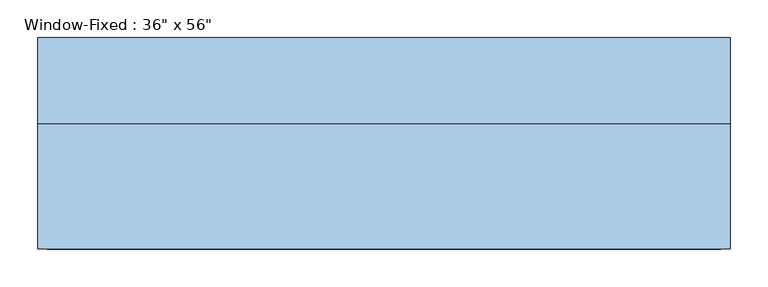
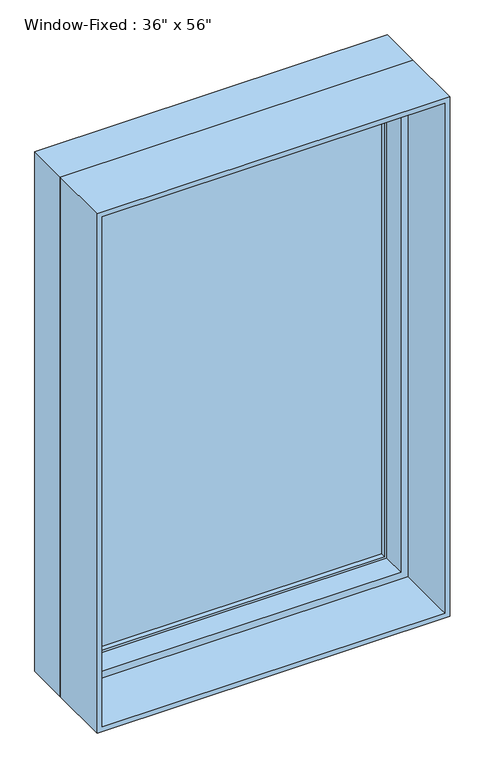
"""IFC4 building model written with IfcOpenShell, lengths in millimetres: window geometry."""

import ifcopenshell
import ifcopenshell.guid

model = None  # the IFC model being written
_history = None  # IfcOwnerHistory: only IFC2X3 demands one
_inside = {}  # id of a spatial element -> (the spatial element, [elements in it])
_under = {}  # id of a project, library or spatial element -> (it, [spatial elements below it])
_declared = {}  # id of a project -> (the project, [libraries it declares])
_typed = {}  # id of a type object -> (the type object, [elements of that type])
_made_of = {}  # id of a material, layer set ... -> (it, [elements and type objects made of it])


def new_model(schema):
    """Start an empty IFC model of exactly this schema.

    Asked for "IFC4X3", IfcOpenShell would pick the latest addendum, in which some entities
    have other attributes; the version numbers below select the first issue.
    IFC2X3 requires an IfcOwnerHistory on every rooted entity: one is made here for all.
    """
    global model, _history
    if schema == "IFC4X3":
        model = ifcopenshell.file(schema_version=(4, 3, 0, 0))
    else:
        model = ifcopenshell.file(schema=schema)
    _inside.clear()
    _under.clear()
    _declared.clear()
    _typed.clear()
    _made_of.clear()
    _history = None
    if model.schema == "IFC2X3":
        org = make("IfcOrganization", Name="unknown")
        user = make(
            "IfcPersonAndOrganization",
            ThePerson=make("IfcPerson", FamilyName="unknown"),
            TheOrganization=org,
        )
        app = make(
            "IfcApplication",
            ApplicationDeveloper=org,
            Version="unknown",
            ApplicationFullName="unknown",
            ApplicationIdentifier="unknown",
        )
        _history = make(
            "IfcOwnerHistory",
            OwningUser=user,
            OwningApplication=app,
            ChangeAction="ADDED",
            CreationDate=0,
        )
    return model


def make(cls, **values):
    """One entity of the class cls with the attributes given. An attribute that is None is left unset."""
    return model.create_entity(
        cls, **{name: value for name, value in values.items() if value is not None}
    )


def rooted(cls, **values):
    """An entity with a GlobalId (a new one), such as an element, a storey or a relation."""
    return make(cls, GlobalId=ifcopenshell.guid.new(), OwnerHistory=_history, **values)


def si_unit(unit_type, name, prefix=None):
    """IfcSIUnit, for example si_unit("LENGTHUNIT", "METRE", prefix="MILLI")."""
    return make("IfcSIUnit", UnitType=unit_type, Prefix=prefix, Name=name)


def assignment(units):
    """IfcUnitAssignment: the units of a project."""
    return None if units is None else make("IfcUnitAssignment", Units=units)


def point(xyz):
    """IfcCartesianPoint."""
    return None if xyz is None else make("IfcCartesianPoint", Coordinates=xyz)


def direction(xyz):
    """IfcDirection."""
    return None if xyz is None else make("IfcDirection", DirectionRatios=xyz)


def frame(location, z_axis=None, x_axis=None):
    """IfcAxis2Placement3D, a coordinate frame: its origin and axes. An axis left out is left unset."""
    return make(
        "IfcAxis2Placement3D",
        Location=point(location),
        Axis=direction(z_axis),
        RefDirection=direction(x_axis),
    )


def origin():
    """The frame at (0, 0, 0) with its axes left unset."""
    return frame((0.0, 0.0, 0.0))


def place(relative_to, where):
    """IfcLocalPlacement: puts the frame where relative to a parent placement (None: the world)."""
    return make(
        "IfcLocalPlacement", PlacementRelTo=relative_to, RelativePlacement=where
    )


def context(
    kind, dimensions, precision=None, world=None, true_north=None, identifier=None
):
    """IfcGeometricRepresentationContext, for example the 3D "Model" context."""
    return make(
        "IfcGeometricRepresentationContext",
        ContextIdentifier=identifier,
        ContextType=kind,
        CoordinateSpaceDimension=dimensions,
        Precision=precision,
        WorldCoordinateSystem=world,
        TrueNorth=true_north,
    )


def project(units=None, contexts=None):
    """IfcProject with its units and contexts."""
    return rooted(
        "IfcProject",
        Name="project",
        RepresentationContexts=contexts,
        UnitsInContext=assignment(units),
    )


def spatial(cls, under=None, at=None, **own):
    """A site, building, storey or space (cls), placed at a placement, below another one or the project."""
    s = rooted(cls, ObjectPlacement=at, **own)
    if under is not None:
        _under.setdefault(under.id(), (under, []))[1].append(s)
    return s


def polyline(points):
    """IfcPolyline through the points."""
    return make("IfcPolyline", Points=[point(p) for p in points])


def outline(outer, holes=None, kind="AREA"):
    """IfcArbitraryClosedProfileDef: a profile drawn as a closed curve; with holes, ...WithVoids."""
    if holes is None:
        return make("IfcArbitraryClosedProfileDef", ProfileType=kind, OuterCurve=outer)
    return make(
        "IfcArbitraryProfileDefWithVoids",
        ProfileType=kind,
        OuterCurve=outer,
        InnerCurves=holes,
    )


def extrude(swept, where, along, depth):
    """IfcExtrudedAreaSolid: the profile swept, set in the frame where, extruded along a direction by depth."""
    return make(
        "IfcExtrudedAreaSolid",
        SweptArea=swept,
        Position=where,
        ExtrudedDirection=direction(along),
        Depth=depth,
    )


def faces_of(points, faces, orient=None, outer=None):
    """IfcFace entities. A face is a list of loops; a loop is a list of indices into points, from 0.

    orient and outer hold one flag for each loop. By default every Orientation is true, the
    first loop of a face is its IfcFaceOuterBound and the others are IfcFaceBound.
    """
    made = []
    for i, loops in enumerate(faces):
        bounds = []
        for j, loop in enumerate(loops):
            is_outer = j == 0 if outer is None else outer[i][j]
            bounds.append(
                make(
                    "IfcFaceOuterBound" if is_outer else "IfcFaceBound",
                    Bound=make("IfcPolyLoop", Polygon=[points[k] for k in loop]),
                    Orientation=True if orient is None else orient[i][j],
                )
            )
        made.append(make("IfcFace", Bounds=bounds))
    return made


def faceted_brep(points, faces, orient=None, outer=None, voids=None):
    """IfcFacetedBrep: a solid bounded by flat faces; with voids (closed shells), ...WithVoids."""
    shared = [point(p) for p in points]
    hull = make("IfcClosedShell", CfsFaces=faces_of(shared, faces, orient, outer))
    if voids is None:
        return make("IfcFacetedBrep", Outer=hull)
    return make(
        "IfcFacetedBrepWithVoids",
        Outer=hull,
        Voids=[
            make(cls, CfsFaces=faces_of(shared, fs, o, b)) for cls, fs, o, b in voids
        ],
    )


def shape(context_of_items, identifier, shape_type, items):
    """IfcShapeRepresentation: the items that make up one representation, for example the "Body"."""
    return make(
        "IfcShapeRepresentation",
        ContextOfItems=context_of_items,
        RepresentationIdentifier=identifier,
        RepresentationType=shape_type,
        Items=items,
    )


def source(mapping_origin, context_of_items, identifier, shape_type, items):
    """IfcRepresentationMap: a shape defined once, which mapped items show again and again."""
    return make(
        "IfcRepresentationMap",
        MappingOrigin=mapping_origin,
        MappedRepresentation=shape(context_of_items, identifier, shape_type, items),
    )


def transform(
    local_origin,
    x_axis=None,
    y_axis=None,
    z_axis=None,
    scale=None,
    scale2=None,
    scale3=None,
    uniform=True,
):
    """IfcCartesianTransformationOperator3D, or its non-uniform kind. x_axis, y_axis, z_axis: its Axis1, 2, 3."""
    if uniform:
        return make(
            "IfcCartesianTransformationOperator3D",
            Axis1=direction(x_axis),
            Axis2=direction(y_axis),
            LocalOrigin=point(local_origin),
            Scale=scale,
            Axis3=direction(z_axis),
        )
    return make(
        "IfcCartesianTransformationOperator3DnonUniform",
        Axis1=direction(x_axis),
        Axis2=direction(y_axis),
        LocalOrigin=point(local_origin),
        Scale=scale,
        Axis3=direction(z_axis),
        Scale2=scale2,
        Scale3=scale3,
    )


def mapped(mapping_source, mapping_target):
    """IfcMappedItem: shows the shape of a source again, moved by a transform."""
    return make(
        "IfcMappedItem", MappingSource=mapping_source, MappingTarget=mapping_target
    )


def made_of(thing, what):
    """Note that an element or type object is made of a material, layer set ...; save() writes the relation."""
    if what is not None:
        _made_of.setdefault(what.id(), (what, []))[1].append(thing)
    return thing


def element(
    cls,
    number,
    at=None,
    inside=None,
    cuts=None,
    type_object=None,
    material=None,
    context=None,
    identifier="Body",
    shape_type=None,
    held_by="IfcProductDefinitionShape",
    body=None,
    shapes=None,
    **own,
):
    """One element of the class cls, such as IfcWall. Its Tag is "e" and its number.

    at: its placement. inside: the storey or other place that contains it. cuts: it is an
    opening in that element (IfcRelVoidsElement). A single representation is given by context,
    identifier, shape_type and body (its items); several are given by shapes. held_by: the class
    of the entity that holds the representations. save() writes the other relations.
    """
    e = rooted(cls, Tag="e%d" % number, ObjectPlacement=at, **own)
    if body is not None:
        shapes = [shape(context, identifier, shape_type, body)]
    if shapes is not None:
        e.Representation = make(held_by, Representations=shapes)
    if inside is not None:
        _inside.setdefault(inside.id(), (inside, []))[1].append(e)
    if cuts is not None:
        rooted(
            "IfcRelVoidsElement", RelatingBuildingElement=cuts, RelatedOpeningElement=e
        )
    if type_object is not None:
        _typed.setdefault(type_object.id(), (type_object, []))[1].append(e)
    return made_of(e, material)


def aggregate(whole, parts):
    """IfcRelAggregates: a whole, such as a stair, and the parts it consists of."""
    return rooted("IfcRelAggregates", RelatingObject=whole, RelatedObjects=parts)


def save(model, path):
    """Write the relations noted so far, then the file.

    IfcRelAggregates (storeys below a building ...), IfcRelContainedInSpatialStructure (elements
    in a storey), IfcRelDefinesByType, IfcRelAssociatesMaterial and IfcRelDeclares: one each for
    every whole, place, type object, material and project.
    """
    for whole, parts in _under.values():
        aggregate(whole, parts)
    for where, things in _inside.values():
        rooted(
            "IfcRelContainedInSpatialStructure",
            RelatedElements=things,
            RelatingStructure=where,
        )
    for kind, things in _typed.values():
        rooted("IfcRelDefinesByType", RelatedObjects=things, RelatingType=kind)
    for what, things in _made_of.values():
        rooted("IfcRelAssociatesMaterial", RelatedObjects=things, RelatingMaterial=what)
    for by, libraries in _declared.values():
        rooted("IfcRelDeclares", RelatingContext=by, RelatedDefinitions=libraries)
    model.write(path)


def window_fe4c84aa(model_context):
    return source(origin(), model_context, "Body", "SolidModel", [
        extrude(outline(polyline([(419.1, 104.775), (419.1, 98.425), (-419.1, 98.425), (-419.1, 104.775), (419.1, 104.775)])), frame((0.0, 0.0, 952.5), z_axis=(0.0, 0.0, 1.0), x_axis=(1.0, 0.0, 0.0)), (0.0, 0.0, 1.0), 1346.2),
        extrude(outline(polyline([(-419.1, 85.725), (-419.1, 92.075), (419.1, 92.075), (419.1, 85.725), (-419.1, 85.725)])), frame((0.0, 0.0, 952.5), z_axis=(0.0, 0.0, 1.0), x_axis=(1.0, 0.0, 0.0)), (0.0, 0.0, 1.0), 1346.2),
        extrude(outline(polyline([(927.1, 444.5), (2324.1, 444.5), (2324.1, -444.5), (927.1, -444.5), (927.1, 444.5)]), holes=[polyline([(952.5, -419.1), (2298.7, -419.1), (2298.7, 419.1), (952.5, 419.1), (952.5, -419.1)])]), frame((0.0, 73.025, 0.0), z_axis=(0.0, 1.0, 0.0), x_axis=(0.0, 0.0, 1.0)), (0.0, 0.0, 1.0), 44.45),
        extrude(outline(polyline([(2336.8, -457.2), (914.4, -457.2), (914.4, 457.2), (2336.8, 457.2), (2336.8, -457.2)]), holes=[polyline([(2324.1, 444.5), (927.1, 444.5), (927.1, -444.5), (2324.1, -444.5), (2324.1, 444.5)])]), frame((0.0, -155.575, 0.0), z_axis=(0.0, 1.0, 0.0), x_axis=(0.0, 0.0, 1.0)), (0.0, 0.0, 1.0), 165.1),
        faceted_brep([(457.2, 9.525, 2336.8), (457.2, 123.825, 2336.8), (-457.2, 123.825, 2336.8), (-457.2, 9.525, 2336.8), (-457.2, 123.825, 914.4), (-457.2, 9.525, 914.4), (457.2, 123.825, 914.4), (457.2, 9.525, 914.4), (425.45, 9.525, 2305.05), (425.45, 9.525, 946.15), (-425.45, 9.525, 946.15), (-425.45, 9.525, 2305.05), (-444.5, 123.825, 2324.1), (-444.5, 123.825, 927.1), (444.5, 123.825, 927.1), (444.5, 123.825, 2324.1), (425.45, 73.025, 2305.05), (-425.45, 73.025, 2305.05), (444.5, 73.025, 2324.1), (-444.5, 73.025, 2324.1), (-425.45, 73.025, 946.15), (-444.5, 73.025, 927.1), (425.45, 73.025, 946.15), (444.5, 73.025, 927.1)], [[[0, 1, 2, 3]], [[3, 2, 4, 5]], [[5, 4, 6, 7]], [[3, 5, 7, 0], [8, 9, 10, 11]], [[7, 6, 1, 0]], [[1, 6, 4, 2], [12, 13, 14, 15]], [[16, 8, 11, 17]], [[15, 18, 19, 12]], [[17, 11, 10, 20]], [[12, 19, 21, 13]], [[20, 10, 9, 22]], [[13, 21, 23, 14]], [[22, 9, 8, 16]], [[18, 23, 21, 19], [17, 20, 22, 16]], [[14, 23, 18, 15]]]),
    ])


if __name__ == "__main__":
    model = new_model("IFC4")
    model_context = context("Model", 3, world=origin())
    ifc_project = project(units=[si_unit("LENGTHUNIT", "METRE", prefix="MILLI")], contexts=[model_context])
    site = spatial("IfcSite", under=ifc_project)
    building = spatial("IfcBuilding", under=site)
    placement = place(None, origin())
    window_shape = window_fe4c84aa(model_context)
    element("IfcWindow", 1, ObjectType="Window-Fixed : 36\" x 56\"", at=placement, inside=building, context=model_context, shape_type="MappedRepresentation", body=[
        mapped(window_shape, transform((0.0, 0.0, 0.0), x_axis=(1.0, 0.0, 0.0), y_axis=(0.0, 1.0, 0.0), z_axis=(0.0, 0.0, 1.0))),
    ])
    save(model, "model.ifc")

# Revit data of these elements
# Type "Window-Fixed : 36\" x 56\""
#   Type Mark = "22"
#   Fire Rating = "0.5h"
#   Assembly Code = "B2020100"
#   Analytic Construction = "Double glazing - domestic"
#   Window Inset [instance default] = 0' - 0"
#   Wall Thickness [instance default] = 0' - 6"
#   Visual Light Transmittance = 0.81
#   Thermal Resistance (R) = 1.8146 (h·ft²·°F)/BTU
#   Solar Heat Gain Coefficient = 0.76
#   Rough Width = 3' - 0 1/2"
#   Rough Height = 4' - 8 1/2"
#   Interior Wall Closure [instance default] = 0' - 2 1/4"
#   Height = 4' - 8"
#   Heat Transfer Coefficient (U) = 0.5511 BTU/(h·ft²·°F)
#   Frame Extension [instance default] = 0' - 0 1/4"
#   Exterior Wall Closure [instance default] = 0' - 1 1/4"
#   Extension Jamb [instance default] = 0' - 2 1/4"
#   Default Sill Height = 3' - 0"
#   Width = 3' - 0"
#   Muntin Visibility = yes
#   Interior Trim Visibility [instance default] = yes
#   Exterior Trim Visibility [instance default] = yes
#   Extension Jamb Visibility [instance default] = yes
#   Muntin Pattern = Muntin Pattern_2x2 : Muntin Pattern_2x2
#   Interior Trim Material = Wood - Stained
#   Interior Trim = Trim-Window-Interior-Flat : Picture Frame
#   Interior Frame Material = Wood - Stained
#   Glass Panel Material = Glass
#   Exterior Trim Material = Clad - White
#   Exterior Trim = Trim-Window-Exterior-Flat : with Sill
#   Exterior Frame Material = Clad - White
#   Wall Closure = (empty or 0)
# Element 1 (IfcWindow, "Window-Fixed : 36\" x 56\"")
#   Window Inset = 0' - 2"
#   Wall Thickness = 1' - 0 1/4"
#   Exterior Wall Closure = 0' - 5 1/2"
#   Extension Jamb = 0' - 6 1/2"
#   Exterior Trim Visibility = no
#   Materials on its faces: "Wood - Stained", "Glass", "Clad - White"
# Materials
#   "Wood - Stained": class "Wood", colour RGB 224 178 126, transparency 0, Cost = 0
#   "Glass": class "Glass", colour RGB 0 128 192, transparency 0.75, Description = "Soda Lime Glass", Cost = 0
#   "Clad - White": class "Wood", colour RGB 242 242 238, transparency 0, Cost = 0
